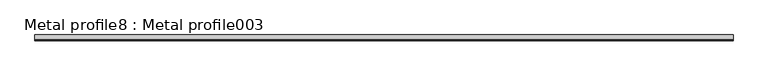
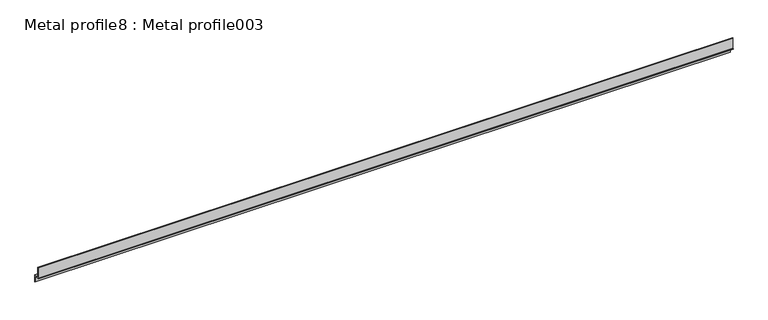
"""IFC4 building model written with IfcOpenShell, lengths in millimetres: proxy geometry, Metal profile8 : Metal profile003."""

from ifc_helpers import new_model, si_unit, frame, origin, place, context, project, spatial, polyline, outline, extrude, source, transform, mapped, element, save


def metal_profile8_metal_profile003_e34a37d0(model_context):
    return source(origin(), model_context, "Body", "SweptSolid", [
        extrude(outline(polyline([(9589.3683229, 36582.096), (9589.3683229, 36601.196), (9574.2702363, 36601.196), (9574.2702363, 36602.466), (9575.0800834, 36602.466), (9575.0800834, 36634.216), (9576.3500834, 36634.216), (9576.3500834, 36602.466), (9590.6383229, 36602.466), (9590.6383229, 36582.096), (9589.3683229, 36582.096)])), frame((3694.2883192, 0.0, 0.0), z_axis=(1.0, 0.0, 0.0), x_axis=(0.0, 1.0, 0.0)), (0.0, 0.0, 1.0), 2000.0),
    ])


if __name__ == "__main__":
    model = new_model("IFC4")
    model_context = context("Model", 3, world=origin())
    ifc_project = project(units=[si_unit("LENGTHUNIT", "METRE", prefix="MILLI")], contexts=[model_context])
    site = spatial("IfcSite", under=ifc_project)
    building = spatial("IfcBuilding", under=site)
    placement = place(None, origin())
    metal_profile8_metal_profile003_shape = metal_profile8_metal_profile003_e34a37d0(model_context)
    element("IfcBuildingElementProxy", 1, Name="Metal profile8 : Metal profile003", ObjectType="Metal profile8 : Metal profile003", at=placement, inside=building, context=model_context, shape_type="MappedRepresentation", body=[
        mapped(metal_profile8_metal_profile003_shape, transform((0.0, 0.0, 0.0), x_axis=(1.0, 0.0, 0.0), y_axis=(0.0, 1.0, 0.0), z_axis=(0.0, 0.0, 1.0))),
    ])
    save(model, "model.ifc")

# Revit data of these elements
# Type "Metal profile8 : Metal profile003"
#   NameOverride = "Metal profile003"
# Element 1 (IfcBuildingElementProxy, "Metal profile8 : Metal profile003")
#   Materials on its faces: "SHADOW Z REVEAL  BEAD"
# Materials
#   "SHADOW Z REVEAL  BEAD": class "Unassigned", colour RGB 251 232 155, transparency 0, Cost = 0
